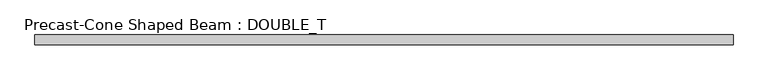
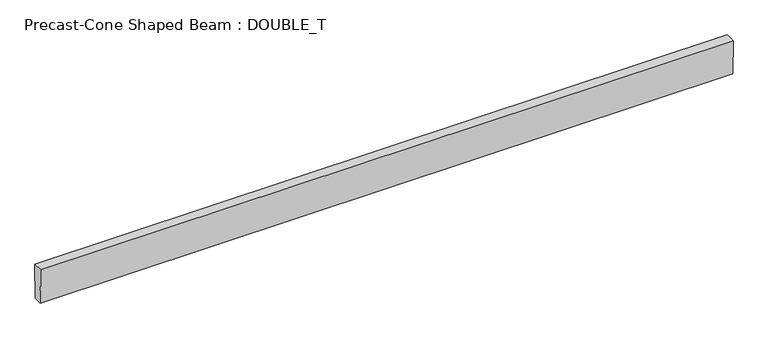
"""IFC4 building model written with IfcOpenShell, lengths in millimetres: beam geometry, Precast-Cone Shaped Beam : DOUBLE_T."""

from ifc_helpers import new_model, si_unit, frame, origin, place, context, project, spatial, polyline, outline, extrude, source, transform, mapped, element, save


def precast_cone_shaped_beam_double_t_e38496ef(model_context):
    return source(origin(), model_context, "Body", "SweptSolid", [
        extrude(outline(polyline([(50.8, -228.6), (-50.8, -228.6), (-63.5, 228.6), (63.5, 228.6), (50.8, -228.6)])), frame((-4311.8111314, 0.0, 0.0), z_axis=(1.0, 0.0, 0.0), x_axis=(0.0, 1.0, 0.0)), (0.0, 0.0, 1.0), 8885.5597628),
    ])


if __name__ == "__main__":
    model = new_model("IFC4")
    model_context = context("Model", 3, world=origin())
    ifc_project = project(units=[si_unit("LENGTHUNIT", "METRE", prefix="MILLI")], contexts=[model_context])
    site = spatial("IfcSite", under=ifc_project)
    building = spatial("IfcBuilding", under=site)
    placement = place(None, origin())
    precast_cone_shaped_beam_double_t_shape = precast_cone_shaped_beam_double_t_e38496ef(model_context)
    element("IfcBeam", 1, ObjectType="Precast-Cone Shaped Beam : DOUBLE_T", at=placement, inside=building, context=model_context, shape_type="MappedRepresentation", body=[
        mapped(precast_cone_shaped_beam_double_t_shape, transform((0.0, 0.0, 0.0), x_axis=(1.0, 0.0, 0.0), y_axis=(0.0, 1.0, 0.0), z_axis=(0.0, 0.0, 1.0))),
    ])
    save(model, "model.ifc")

# Revit data of these elements
# Type "Precast-Cone Shaped Beam : DOUBLE_T"
#   Top Width = 0' - 5"
#   Tie Rod Weight [instance default] = 30
#   Tie Rod W [instance default] = 0.0660938 kip
#   Single Rebar Weight [instance default] = 50
#   Single Rebar W [instance default] = 0.110156 kip
#   Rebar Grids Weight [instance default] = 100
#   Rebar Grids W [instance default] = 0.220313 kip
#   Depth = 1' - 6"
#   Bottom Width = 0' - 4"
#   Length [instance default] = 5' - 0"
#   Structural Material [instance default] = Concrete, Precast
#   Assembly Code = ""
# Element 1 (IfcBeam, "Precast-Cone Shaped Beam : DOUBLE_T")
#   Length = 29' - 3.51269"
#   Structural Material = Concrete - Precast Concrete - Normal Weight Concrete - 5 ksi
#   Materials on its faces: "Concrete - Precast Concrete - Normal Weight Concrete - 5 ksi"
# Materials
#   "Concrete, Precast": class "Concrete", colour RGB 198 187 187, transparency 0, Description = "Precast concrete", Cost = 0
#   "Concrete - Precast Concrete - Normal Weight Concrete - 5 ksi": class "Concrete", colour RGB 198 187 187, transparency 0, Cost = 0
